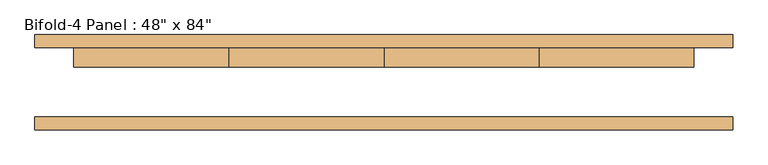
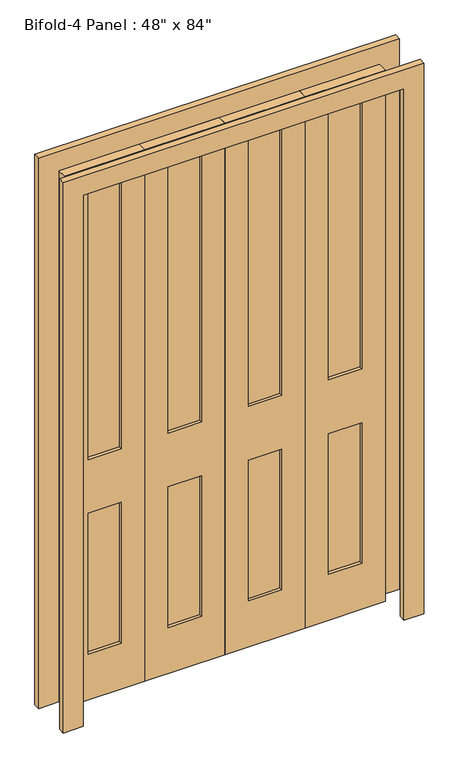
"""IFC4 building model written with IfcOpenShell, lengths in millimetres: door geometry."""

from ifc_helpers import new_model, si_unit, frame, origin, place, context, project, spatial, polyline, outline, extrude, source, transform, mapped, element, save


def door_ad0b5cc3(model_context):
    return source(origin(), model_context, "Body", "SweptSolid", [
        extrude(outline(polyline([(393.7, 55.5625), (520.7, 55.5625), (520.7, 42.8625), (393.7, 42.8625), (393.7, 55.5625)])), frame((0.0, 0.0, 965.2), z_axis=(0.0, 0.0, 1.0), x_axis=(1.0, 0.0, 0.0)), (0.0, 0.0, 1.0), 1085.85),
        extrude(outline(polyline([(393.7, 55.5625), (520.7, 55.5625), (520.7, 42.8625), (393.7, 42.8625), (393.7, 55.5625)])), frame((0.0, 0.0, 184.15), z_axis=(0.0, 0.0, 1.0), x_axis=(1.0, 0.0, 0.0)), (0.0, 0.0, 1.0), 565.15),
        extrude(outline(polyline([(88.9, 55.5625), (215.9, 55.5625), (215.9, 42.8625), (88.9, 42.8625), (88.9, 55.5625)])), frame((0.0, 0.0, 965.2), z_axis=(0.0, 0.0, 1.0), x_axis=(1.0, 0.0, 0.0)), (0.0, 0.0, 1.0), 1085.85),
        extrude(outline(polyline([(88.9, 55.5625), (215.9, 55.5625), (215.9, 42.8625), (88.9, 42.8625), (88.9, 55.5625)])), frame((0.0, 0.0, 184.15), z_axis=(0.0, 0.0, 1.0), x_axis=(1.0, 0.0, 0.0)), (0.0, 0.0, 1.0), 565.15),
        extrude(outline(polyline([(-215.9, 55.5625), (-88.9, 55.5625), (-88.9, 42.8625), (-215.9, 42.8625), (-215.9, 55.5625)])), frame((0.0, 0.0, 184.15), z_axis=(0.0, 0.0, 1.0), x_axis=(1.0, 0.0, 0.0)), (0.0, 0.0, 1.0), 565.15),
        extrude(outline(polyline([(-215.9, 55.5625), (-88.9, 55.5625), (-88.9, 42.8625), (-215.9, 42.8625), (-215.9, 55.5625)])), frame((0.0, 0.0, 965.2), z_axis=(0.0, 0.0, 1.0), x_axis=(1.0, 0.0, 0.0)), (0.0, 0.0, 1.0), 1085.85),
        extrude(outline(polyline([(-520.7, 55.5625), (-393.7, 55.5625), (-393.7, 42.8625), (-520.7, 42.8625), (-520.7, 55.5625)])), frame((0.0, 0.0, 965.2), z_axis=(0.0, 0.0, 1.0), x_axis=(1.0, 0.0, 0.0)), (0.0, 0.0, 1.0), 1085.85),
        extrude(outline(polyline([(-520.7, 55.5625), (-393.7, 55.5625), (-393.7, 42.8625), (-520.7, 42.8625), (-520.7, 55.5625)])), frame((0.0, 0.0, 184.15), z_axis=(0.0, 0.0, 1.0), x_axis=(1.0, 0.0, 0.0)), (0.0, 0.0, 1.0), 565.15),
        extrude(outline(polyline([(0.0, 685.8), (2209.8, 685.8), (2209.8, -685.8), (0.0, -685.8), (0.0, -609.6), (2133.6, -609.6), (2133.6, 609.6), (0.0, 609.6), (0.0, 685.8)])), frame((0.0, -93.6625, 0.0), z_axis=(0.0, 1.0, 0.0), x_axis=(0.0, 0.0, 1.0)), (0.0, 0.0, 1.0), 25.4),
        extrude(outline(polyline([(0.0, 685.8), (2209.8, 685.8), (2209.8, -685.8), (0.0, -685.8), (0.0, -609.6), (2133.6, -609.6), (2133.6, 609.6), (0.0, 609.6), (0.0, 685.8)])), frame((0.0, 68.2625, 0.0), z_axis=(0.0, 1.0, 0.0), x_axis=(0.0, 0.0, 1.0)), (0.0, 0.0, 1.0), 25.4),
        extrude(outline(polyline([(0.0, -609.6), (0.0, -304.8), (2133.6, -304.8), (2133.6, -609.6), (0.0, -609.6)]), holes=[polyline([(2051.05, -520.7), (2051.05, -393.7), (965.2, -393.7), (965.2, -520.7), (2051.05, -520.7)]), polyline([(749.3, -520.7), (749.3, -393.7), (184.15, -393.7), (184.15, -520.7), (749.3, -520.7)])]), frame((0.0, 30.1625, 0.0), z_axis=(0.0, 1.0, 0.0), x_axis=(0.0, 0.0, 1.0)), (0.0, 0.0, 1.0), 38.1),
        extrude(outline(polyline([(0.0, -304.8), (0.0, 0.0), (2133.6, 0.0), (2133.6, -304.8), (0.0, -304.8)]), holes=[polyline([(2051.05, -215.9), (2051.05, -88.9), (965.2, -88.9), (965.2, -215.9), (2051.05, -215.9)]), polyline([(749.3, -215.9), (749.3, -88.9), (184.15, -88.9), (184.15, -215.9), (749.3, -215.9)])]), frame((0.0, 30.1625, 0.0), z_axis=(0.0, 1.0, 0.0), x_axis=(0.0, 0.0, 1.0)), (0.0, 0.0, 1.0), 38.1),
        extrude(outline(polyline([(0.0, 0.0), (0.0, 304.8), (2133.6, 304.8), (2133.6, 0.0), (0.0, 0.0)]), holes=[polyline([(2051.05, 88.9), (2051.05, 215.9), (965.2, 215.9), (965.2, 88.9), (2051.05, 88.9)]), polyline([(749.3, 88.9), (749.3, 215.9), (184.15, 215.9), (184.15, 88.9), (749.3, 88.9)])]), frame((0.0, 30.1625, 0.0), z_axis=(0.0, 1.0, 0.0), x_axis=(0.0, 0.0, 1.0)), (0.0, 0.0, 1.0), 38.1),
        extrude(outline(polyline([(0.0, 304.8), (0.0, 609.6), (2133.6, 609.6), (2133.6, 304.8), (0.0, 304.8)]), holes=[polyline([(2051.05, 393.7), (2051.05, 520.7), (965.2, 520.7), (965.2, 393.7), (2051.05, 393.7)]), polyline([(749.3, 393.7), (749.3, 520.7), (184.15, 520.7), (184.15, 393.7), (749.3, 393.7)])]), frame((0.0, 30.1625, 0.0), z_axis=(0.0, 1.0, 0.0), x_axis=(0.0, 0.0, 1.0)), (0.0, 0.0, 1.0), 38.1),
    ])


if __name__ == "__main__":
    model = new_model("IFC4")
    model_context = context("Model", 3, world=origin())
    ifc_project = project(units=[si_unit("LENGTHUNIT", "METRE", prefix="MILLI")], contexts=[model_context])
    site = spatial("IfcSite", under=ifc_project)
    building = spatial("IfcBuilding", under=site)
    placement = place(None, origin())
    door_shape = door_ad0b5cc3(model_context)
    element("IfcDoor", 1, ObjectType="Bifold-4 Panel : 48\" x 84\"", at=placement, inside=building, context=model_context, shape_type="MappedRepresentation", body=[
        mapped(door_shape, transform((0.0, 0.0, 0.0), x_axis=(1.0, 0.0, 0.0), y_axis=(0.0, 1.0, 0.0), z_axis=(0.0, 0.0, 1.0))),
    ])
    save(model, "model.ifc")

# Revit data of these elements
# Type "Bifold-4 Panel : 48\" x 84\""
#   Type Mark = "38"
#   Assembly Code = "C1020"
#   Thickness = 0' - 1 1/2"
#   Height = 7' - 0"
#   Trim Width = 0' - 3"
#   Width = 4' - 0"
#   Door Material = Door - Panel
#   Frame Material = Door - Frame
#   Function = (empty or 0)
#   Description = (empty or 0)
#   Wall Closure = (empty or 0)
# Element 1 (IfcDoor, "Bifold-4 Panel : 48\" x 84\"")
#   Materials on its faces: "Door - Panel", "Door - Frame"
# Materials
#   "Door - Panel": class "Wood", colour RGB 210 159 95, transparency 0, Cost = 0
#   "Door - Frame": class "Miscellaneous", colour RGB 118 70 51, transparency 0, Cost = 0
